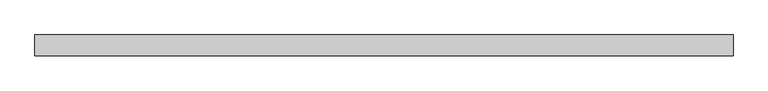
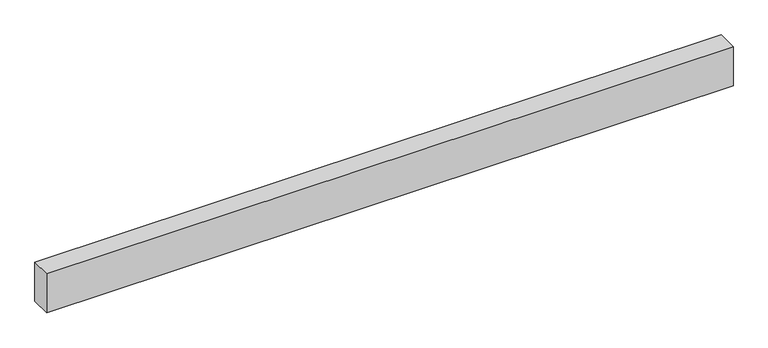
"""IFC4 building model written with IfcOpenShell, lengths in millimetres: beam geometry, Madeira de lei : Berço 6x12cm."""

import ifcopenshell
import ifcopenshell.guid

model = None  # the IFC model being written
_history = None  # IfcOwnerHistory: only IFC2X3 demands one
_inside = {}  # id of a spatial element -> (the spatial element, [elements in it])
_under = {}  # id of a project, library or spatial element -> (it, [spatial elements below it])
_declared = {}  # id of a project -> (the project, [libraries it declares])
_typed = {}  # id of a type object -> (the type object, [elements of that type])
_made_of = {}  # id of a material, layer set ... -> (it, [elements and type objects made of it])


def new_model(schema):
    """Start an empty IFC model of exactly this schema.

    Asked for "IFC4X3", IfcOpenShell would pick the latest addendum, in which some entities
    have other attributes; the version numbers below select the first issue.
    IFC2X3 requires an IfcOwnerHistory on every rooted entity: one is made here for all.
    """
    global model, _history
    if schema == "IFC4X3":
        model = ifcopenshell.file(schema_version=(4, 3, 0, 0))
    else:
        model = ifcopenshell.file(schema=schema)
    _inside.clear()
    _under.clear()
    _declared.clear()
    _typed.clear()
    _made_of.clear()
    _history = None
    if model.schema == "IFC2X3":
        org = make("IfcOrganization", Name="unknown")
        user = make(
            "IfcPersonAndOrganization",
            ThePerson=make("IfcPerson", FamilyName="unknown"),
            TheOrganization=org,
        )
        app = make(
            "IfcApplication",
            ApplicationDeveloper=org,
            Version="unknown",
            ApplicationFullName="unknown",
            ApplicationIdentifier="unknown",
        )
        _history = make(
            "IfcOwnerHistory",
            OwningUser=user,
            OwningApplication=app,
            ChangeAction="ADDED",
            CreationDate=0,
        )
    return model


def make(cls, **values):
    """One entity of the class cls with the attributes given. An attribute that is None is left unset."""
    return model.create_entity(
        cls, **{name: value for name, value in values.items() if value is not None}
    )


def rooted(cls, **values):
    """An entity with a GlobalId (a new one), such as an element, a storey or a relation."""
    return make(cls, GlobalId=ifcopenshell.guid.new(), OwnerHistory=_history, **values)


def si_unit(unit_type, name, prefix=None):
    """IfcSIUnit, for example si_unit("LENGTHUNIT", "METRE", prefix="MILLI")."""
    return make("IfcSIUnit", UnitType=unit_type, Prefix=prefix, Name=name)


def assignment(units):
    """IfcUnitAssignment: the units of a project."""
    return None if units is None else make("IfcUnitAssignment", Units=units)


def point(xyz):
    """IfcCartesianPoint."""
    return None if xyz is None else make("IfcCartesianPoint", Coordinates=xyz)


def direction(xyz):
    """IfcDirection."""
    return None if xyz is None else make("IfcDirection", DirectionRatios=xyz)


def frame(location, z_axis=None, x_axis=None):
    """IfcAxis2Placement3D, a coordinate frame: its origin and axes. An axis left out is left unset."""
    return make(
        "IfcAxis2Placement3D",
        Location=point(location),
        Axis=direction(z_axis),
        RefDirection=direction(x_axis),
    )


def origin():
    """The frame at (0, 0, 0) with its axes left unset."""
    return frame((0.0, 0.0, 0.0))


def place(relative_to, where):
    """IfcLocalPlacement: puts the frame where relative to a parent placement (None: the world)."""
    return make(
        "IfcLocalPlacement", PlacementRelTo=relative_to, RelativePlacement=where
    )


def context(
    kind, dimensions, precision=None, world=None, true_north=None, identifier=None
):
    """IfcGeometricRepresentationContext, for example the 3D "Model" context."""
    return make(
        "IfcGeometricRepresentationContext",
        ContextIdentifier=identifier,
        ContextType=kind,
        CoordinateSpaceDimension=dimensions,
        Precision=precision,
        WorldCoordinateSystem=world,
        TrueNorth=true_north,
    )


def project(units=None, contexts=None):
    """IfcProject with its units and contexts."""
    return rooted(
        "IfcProject",
        Name="project",
        RepresentationContexts=contexts,
        UnitsInContext=assignment(units),
    )


def spatial(cls, under=None, at=None, **own):
    """A site, building, storey or space (cls), placed at a placement, below another one or the project."""
    s = rooted(cls, ObjectPlacement=at, **own)
    if under is not None:
        _under.setdefault(under.id(), (under, []))[1].append(s)
    return s


def polyline(points):
    """IfcPolyline through the points."""
    return make("IfcPolyline", Points=[point(p) for p in points])


def outline(outer, holes=None, kind="AREA"):
    """IfcArbitraryClosedProfileDef: a profile drawn as a closed curve; with holes, ...WithVoids."""
    if holes is None:
        return make("IfcArbitraryClosedProfileDef", ProfileType=kind, OuterCurve=outer)
    return make(
        "IfcArbitraryProfileDefWithVoids",
        ProfileType=kind,
        OuterCurve=outer,
        InnerCurves=holes,
    )


def extrude(swept, where, along, depth):
    """IfcExtrudedAreaSolid: the profile swept, set in the frame where, extruded along a direction by depth."""
    return make(
        "IfcExtrudedAreaSolid",
        SweptArea=swept,
        Position=where,
        ExtrudedDirection=direction(along),
        Depth=depth,
    )


def shape(context_of_items, identifier, shape_type, items):
    """IfcShapeRepresentation: the items that make up one representation, for example the "Body"."""
    return make(
        "IfcShapeRepresentation",
        ContextOfItems=context_of_items,
        RepresentationIdentifier=identifier,
        RepresentationType=shape_type,
        Items=items,
    )


def source(mapping_origin, context_of_items, identifier, shape_type, items):
    """IfcRepresentationMap: a shape defined once, which mapped items show again and again."""
    return make(
        "IfcRepresentationMap",
        MappingOrigin=mapping_origin,
        MappedRepresentation=shape(context_of_items, identifier, shape_type, items),
    )


def transform(
    local_origin,
    x_axis=None,
    y_axis=None,
    z_axis=None,
    scale=None,
    scale2=None,
    scale3=None,
    uniform=True,
):
    """IfcCartesianTransformationOperator3D, or its non-uniform kind. x_axis, y_axis, z_axis: its Axis1, 2, 3."""
    if uniform:
        return make(
            "IfcCartesianTransformationOperator3D",
            Axis1=direction(x_axis),
            Axis2=direction(y_axis),
            LocalOrigin=point(local_origin),
            Scale=scale,
            Axis3=direction(z_axis),
        )
    return make(
        "IfcCartesianTransformationOperator3DnonUniform",
        Axis1=direction(x_axis),
        Axis2=direction(y_axis),
        LocalOrigin=point(local_origin),
        Scale=scale,
        Axis3=direction(z_axis),
        Scale2=scale2,
        Scale3=scale3,
    )


def mapped(mapping_source, mapping_target):
    """IfcMappedItem: shows the shape of a source again, moved by a transform."""
    return make(
        "IfcMappedItem", MappingSource=mapping_source, MappingTarget=mapping_target
    )


def made_of(thing, what):
    """Note that an element or type object is made of a material, layer set ...; save() writes the relation."""
    if what is not None:
        _made_of.setdefault(what.id(), (what, []))[1].append(thing)
    return thing


def element(
    cls,
    number,
    at=None,
    inside=None,
    cuts=None,
    type_object=None,
    material=None,
    context=None,
    identifier="Body",
    shape_type=None,
    held_by="IfcProductDefinitionShape",
    body=None,
    shapes=None,
    **own,
):
    """One element of the class cls, such as IfcWall. Its Tag is "e" and its number.

    at: its placement. inside: the storey or other place that contains it. cuts: it is an
    opening in that element (IfcRelVoidsElement). A single representation is given by context,
    identifier, shape_type and body (its items); several are given by shapes. held_by: the class
    of the entity that holds the representations. save() writes the other relations.
    """
    e = rooted(cls, Tag="e%d" % number, ObjectPlacement=at, **own)
    if body is not None:
        shapes = [shape(context, identifier, shape_type, body)]
    if shapes is not None:
        e.Representation = make(held_by, Representations=shapes)
    if inside is not None:
        _inside.setdefault(inside.id(), (inside, []))[1].append(e)
    if cuts is not None:
        rooted(
            "IfcRelVoidsElement", RelatingBuildingElement=cuts, RelatedOpeningElement=e
        )
    if type_object is not None:
        _typed.setdefault(type_object.id(), (type_object, []))[1].append(e)
    return made_of(e, material)


def aggregate(whole, parts):
    """IfcRelAggregates: a whole, such as a stair, and the parts it consists of."""
    return rooted("IfcRelAggregates", RelatingObject=whole, RelatedObjects=parts)


def save(model, path):
    """Write the relations noted so far, then the file.

    IfcRelAggregates (storeys below a building ...), IfcRelContainedInSpatialStructure (elements
    in a storey), IfcRelDefinesByType, IfcRelAssociatesMaterial and IfcRelDeclares: one each for
    every whole, place, type object, material and project.
    """
    for whole, parts in _under.values():
        aggregate(whole, parts)
    for where, things in _inside.values():
        rooted(
            "IfcRelContainedInSpatialStructure",
            RelatedElements=things,
            RelatingStructure=where,
        )
    for kind, things in _typed.values():
        rooted("IfcRelDefinesByType", RelatedObjects=things, RelatingType=kind)
    for what, things in _made_of.values():
        rooted("IfcRelAssociatesMaterial", RelatedObjects=things, RelatingMaterial=what)
    for by, libraries in _declared.values():
        rooted("IfcRelDeclares", RelatingContext=by, RelatedDefinitions=libraries)
    model.write(path)


def beam_fe4ddbad(model_context):
    return source(origin(), model_context, "Body", "SweptSolid", [
        extrude(outline(polyline([(998.8971968, 30.0), (998.8971968, -30.0), (-998.8971974, -30.0), (-998.8971974, 30.0), (998.8971968, 30.0)])), frame((0.0, 0.0, -60.0), z_axis=(0.0, 0.0, 1.0), x_axis=(1.0, 0.0, 0.0)), (0.0, 0.0, 1.0), 120.0),
    ])


if __name__ == "__main__":
    model = new_model("IFC4")
    model_context = context("Model", 3, world=origin())
    ifc_project = project(units=[si_unit("LENGTHUNIT", "METRE", prefix="MILLI")], contexts=[model_context])
    site = spatial("IfcSite", under=ifc_project)
    building = spatial("IfcBuilding", under=site)
    placement = place(None, origin())
    beam_shape = beam_fe4ddbad(model_context)
    element("IfcBeam", 1, ObjectType="Madeira de lei : Berço 6x12cm", at=placement, inside=building, context=model_context, shape_type="MappedRepresentation", body=[
        mapped(beam_shape, transform((0.0, 0.0, 0.0), x_axis=(1.0, 0.0, 0.0), y_axis=(0.0, 1.0, 0.0), z_axis=(0.0, 0.0, 1.0))),
    ])
    save(model, "model.ifc")

# Revit data of these elements
# Type "Madeira de lei : Berço 6x12cm"
#   A = 0.02 m²
#   Length [instance default] = 1.524 m
#   b = 0.06 m
#   d = 0.12 m
#   Structural Material [instance default] = none
#   Assembly Code = ""
# Element 1 (IfcBeam, "Madeira de lei : Berço 6x12cm")
#   Structural Material = .MADEIRAMENTO
#   Materials on its faces: ".MADEIRAMENTO"
# Materials
#   ".MADEIRAMENTO": class ".CC_MADEIRAS", colour RGB 212 179 113, transparency 0, Cost = 0
